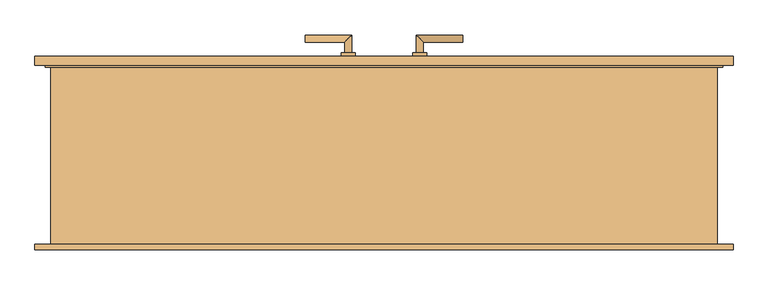
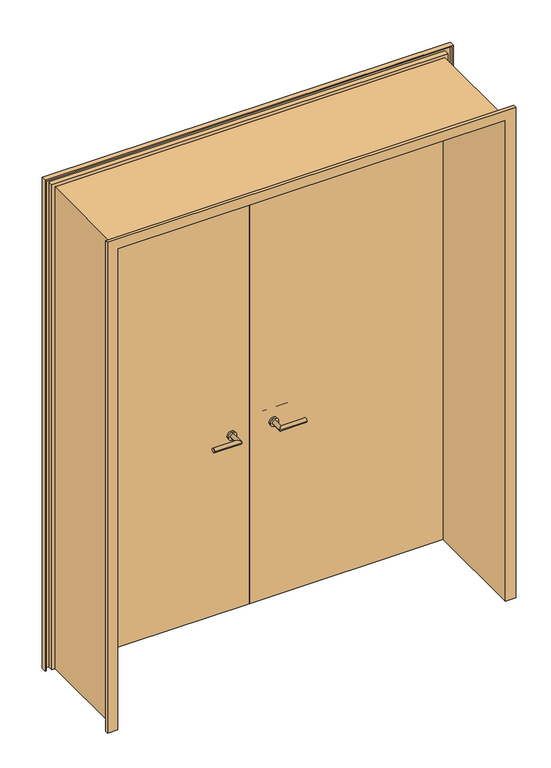
"""IFC4 building model written with IfcOpenShell, lengths in millimetres: door geometry, Drehflügel 2-flg - Stahlzarge : Holztüre 2 flg.1.9x 2.45."""

from ifc_helpers import new_model, si_unit, point, frame, frame_2d, origin, place, context, project, spatial, polyline, circle_curve, ellipse_curve, trimmed, segment, composite_curve, outline, extrude, faceted_brep, source, transform, mapped, element, save
from ifc_brep_helpers import plane_surface, cylinder_surface, advanced_brep


def door_70b3f378(model_context):
    return source(origin(), model_context, "Body", "SolidModel", [
        advanced_brep(
        [(-90.0, 239.4346141, 1000.0), (-110.0, 239.4346141, 1000.0), (-110.0, 189.4346141, 1000.0), (-90.0, 169.4346141, 1000.0), (-220.0, 169.4346141, 1000.0), (-220.0, 189.4346141, 1000.0)],
        [
            (0, 1, circle_curve(frame((-100.0, 239.4346141, 1000.0), z_axis=(0.0, 1.0, 0.0), x_axis=(-1.0, 0.0, 0.0)), 10.0)),
            (1, 0, circle_curve(frame((-100.0, 239.4346141, 1000.0), z_axis=(0.0, 1.0, 0.0), x_axis=(-1.0, 0.0, 0.0)), 10.0)),
            (1, 2),
            (2, 3, ellipse_curve(frame((-100.0, 179.4346141, 1000.0), z_axis=(0.7071067811865385, 0.7071067811865565, 0.0), x_axis=(-0.7071067811865563, 0.7071067811865386, 0.0)), 14.1421356, 10.0)),
            (3, 0),
            (3, 2, ellipse_curve(frame((-100.0, 179.4346141, 1000.0), z_axis=(0.7071067811865385, 0.7071067811865565, 0.0), x_axis=(-0.7071067811865563, 0.7071067811865386, 0.0)), 14.1421356, 10.0)),
            (4, 5, circle_curve(frame((-220.0, 179.4346141, 1000.0), z_axis=(-1.0, 0.0, 0.0), x_axis=(0.0, 1.0, 0.0)), 10.0)),
            (5, 4, circle_curve(frame((-220.0, 179.4346141, 1000.0), z_axis=(-1.0, 0.0, 0.0), x_axis=(0.0, 1.0, 0.0)), 10.0)),
            (2, 5),
            (4, 3),
        ],
        [
            plane_surface(frame((-100.0, 239.4346141, -287.7526403), z_axis=(0.0, 1.0, 0.0), x_axis=(0.0, 0.0, 1.0))),
            cylinder_surface(frame((-100.0, 239.4346141, 1000.0), z_axis=(0.0, 1.0, 0.0), x_axis=(-1.0, 0.0, 0.0)), 10.0),
            plane_surface(frame((-220.0, 179.4346141, -287.7526403), z_axis=(-1.0, 0.0, 0.0), x_axis=(0.0, 0.0, 1.0))),
            cylinder_surface(frame((-100.0, 179.4346141, 1000.0), z_axis=(1.0, 0.0, 0.0), x_axis=(0.0, 1.0, 0.0)), 10.0),
        ],
        [
            (0, [[1, 2]]),
            (1, [[3, 4, 5, -2]]),
            (1, [[-5, 6, -3, -1]]),
            (2, [[7, 8]]),
            (3, [[9, -7, 10, -4]]),
            (3, [[-10, -8, -9, -6]]),
        ],
    ),
        advanced_brep(
        [(-110.0, 299.4346141, 1000.0), (-90.0, 299.4346141, 1000.0), (-90.0, 349.4346141, 1000.0), (-110.0, 329.4346141, 1000.0), (-220.0, 329.4346141, 1000.0), (-220.0, 349.4346141, 1000.0)],
        [
            (0, 1, circle_curve(frame((-100.0, 299.4346141, 1000.0), z_axis=(0.0, -1.0, 0.0), x_axis=(1.0, 0.0, 0.0)), 10.0)),
            (1, 0, circle_curve(frame((-100.0, 299.4346141, 1000.0), z_axis=(0.0, -1.0, 0.0), x_axis=(1.0, 0.0, 0.0)), 10.0)),
            (1, 2),
            (2, 3, ellipse_curve(frame((-100.0, 339.4346141, 1000.0), z_axis=(0.7071067811865475, -0.7071067811865475, 0.0), x_axis=(-0.7071067811865474, -0.7071067811865476, 0.0)), 14.1421356, 10.0)),
            (3, 0),
            (3, 2, ellipse_curve(frame((-100.0, 339.4346141, 1000.0), z_axis=(0.7071067811865475, -0.7071067811865475, 0.0), x_axis=(-0.7071067811865474, -0.7071067811865476, 0.0)), 14.1421356, 10.0)),
            (4, 5, circle_curve(frame((-220.0, 339.4346141, 1000.0), z_axis=(-1.0, 0.0, 0.0), x_axis=(0.0, 1.0, 0.0)), 10.0)),
            (5, 4, circle_curve(frame((-220.0, 339.4346141, 1000.0), z_axis=(-1.0, 0.0, 0.0), x_axis=(0.0, 1.0, 0.0)), 10.0)),
            (2, 5),
            (4, 3),
        ],
        [
            plane_surface(frame((-100.0, 299.4346141, -287.7526403), z_axis=(0.0, -1.0, 0.0), x_axis=(0.0, 0.0, 1.0))),
            cylinder_surface(frame((-100.0, 299.4346141, 1000.0), z_axis=(0.0, -1.0, 0.0), x_axis=(1.0, 0.0, 0.0)), 10.0),
            plane_surface(frame((-220.0, 339.4346141, -287.7526403), z_axis=(-1.0, 0.0, 0.0), x_axis=(0.0, 0.0, 1.0))),
            cylinder_surface(frame((-100.0, 339.4346141, 1000.0), z_axis=(1.0, 0.0, 0.0), x_axis=(0.0, 1.0, 0.0)), 10.0),
        ],
        [
            (0, [[1, 2]]),
            (1, [[3, 4, 5, -2]]),
            (1, [[-5, 6, -3, -1]]),
            (2, [[7, 8]]),
            (3, [[9, -7, 10, -4]]),
            (3, [[-10, -8, -9, -6]]),
        ],
    ),
        extrude(outline(composite_curve([segment(trimmed(circle_curve(frame_2d((1000.0, -100.0)), 20.0), [point((1000.0, -80.0))], [point((1000.0, -120.0))], False, "CARTESIAN"), True, "CONTINUOUS"), segment(trimmed(circle_curve(frame_2d((1000.0, -100.0)), 20.0), [point((1000.0, -120.0))], [point((1000.0, -80.0))], False, "CARTESIAN"), True, "CONTINUOUS")], self_intersect=False)), frame((0.0, 229.4346141, 0.0), z_axis=(0.0, 1.0, 0.0), x_axis=(0.0, 0.0, 1.0)), (0.0, 0.0, 1.0), 10.0),
        extrude(outline(composite_curve([segment(trimmed(circle_curve(frame_2d((1000.0, -100.0)), 20.0), [point((1000.0, -80.0))], [point((1000.0, -120.0))], False, "CARTESIAN"), True, "CONTINUOUS"), segment(trimmed(circle_curve(frame_2d((1000.0, -100.0)), 20.0), [point((1000.0, -120.0))], [point((1000.0, -80.0))], False, "CARTESIAN"), True, "CONTINUOUS")], self_intersect=False)), frame((0.0, 289.4346141, 0.0), z_axis=(0.0, 1.0, 0.0), x_axis=(0.0, 0.0, 1.0)), (0.0, 0.0, 1.0), 10.0),
        advanced_brep(
        [(90.0, 239.4346141, 1000.0), (110.0, 239.4346141, 1000.0), (90.0, 169.4346141, 1000.0), (110.0, 189.4346141, 1000.0), (220.0, 169.4346141, 1000.0), (220.0, 189.4346141, 1000.0)],
        [
            (0, 1, circle_curve(frame((100.0, 239.4346141, 1000.0), z_axis=(0.0, 1.0, 0.0), x_axis=(1.0, 0.0, 0.0)), 10.0)),
            (1, 0, circle_curve(frame((100.0, 239.4346141, 1000.0), z_axis=(0.0, 1.0, 0.0), x_axis=(1.0, 0.0, 0.0)), 10.0)),
            (0, 2),
            (2, 3, ellipse_curve(frame((100.0, 179.4346141, 1000.0), z_axis=(-0.7071067811865385, 0.7071067811865565, 0.0), x_axis=(0.7071067811865563, 0.7071067811865386, 0.0)), 14.1421356, 10.0)),
            (3, 1),
            (3, 2, ellipse_curve(frame((100.0, 179.4346141, 1000.0), z_axis=(-0.7071067811865385, 0.7071067811865565, 0.0), x_axis=(0.7071067811865563, 0.7071067811865386, 0.0)), 14.1421356, 10.0)),
            (4, 5, circle_curve(frame((220.0, 179.4346141, 1000.0), z_axis=(1.0, 0.0, 0.0), x_axis=(0.0, 1.0, 0.0)), 10.0)),
            (5, 4, circle_curve(frame((220.0, 179.4346141, 1000.0), z_axis=(1.0, 0.0, 0.0), x_axis=(0.0, 1.0, 0.0)), 10.0)),
            (2, 4),
            (5, 3),
        ],
        [
            plane_surface(frame((100.0, 239.4346141, -287.7526403), z_axis=(0.0, 1.0, 0.0), x_axis=(0.0, 0.0, 1.0))),
            cylinder_surface(frame((100.0, 239.4346141, 1000.0), z_axis=(0.0, 1.0, 0.0), x_axis=(1.0, 0.0, 0.0)), 10.0),
            plane_surface(frame((220.0, 179.4346141, -287.7526403), z_axis=(1.0, 0.0, 0.0), x_axis=(0.0, 0.0, 1.0))),
            cylinder_surface(frame((100.0, 179.4346141, 1000.0), z_axis=(-1.0, 0.0, 0.0), x_axis=(0.0, 1.0, 0.0)), 10.0),
        ],
        [
            (0, [[1, 2]]),
            (1, [[-1, 3, 4, 5]]),
            (1, [[-2, -5, 6, -3]]),
            (2, [[7, 8]]),
            (3, [[-4, 9, -8, 10]]),
            (3, [[-6, -10, -7, -9]]),
        ],
    ),
        advanced_brep(
        [(110.0, 299.4346141, 1000.0), (90.0, 299.4346141, 1000.0), (110.0, 329.4346141, 1000.0), (90.0, 349.4346141, 1000.0), (220.0, 329.4346141, 1000.0), (220.0, 349.4346141, 1000.0)],
        [
            (0, 1, circle_curve(frame((100.0, 299.4346141, 1000.0), z_axis=(0.0, -1.0, 0.0), x_axis=(-1.0, 0.0, 0.0)), 10.0)),
            (1, 0, circle_curve(frame((100.0, 299.4346141, 1000.0), z_axis=(0.0, -1.0, 0.0), x_axis=(-1.0, 0.0, 0.0)), 10.0)),
            (0, 2),
            (2, 3, ellipse_curve(frame((100.0, 339.4346141, 1000.0), z_axis=(-0.7071067811865475, -0.7071067811865475, 0.0), x_axis=(0.7071067811865474, -0.7071067811865476, 0.0)), 14.1421356, 10.0)),
            (3, 1),
            (3, 2, ellipse_curve(frame((100.0, 339.4346141, 1000.0), z_axis=(-0.7071067811865475, -0.7071067811865475, 0.0), x_axis=(0.7071067811865474, -0.7071067811865476, 0.0)), 14.1421356, 10.0)),
            (4, 5, circle_curve(frame((220.0, 339.4346141, 1000.0), z_axis=(1.0, 0.0, 0.0), x_axis=(0.0, 1.0, 0.0)), 10.0)),
            (5, 4, circle_curve(frame((220.0, 339.4346141, 1000.0), z_axis=(1.0, 0.0, 0.0), x_axis=(0.0, 1.0, 0.0)), 10.0)),
            (2, 4),
            (5, 3),
        ],
        [
            plane_surface(frame((100.0, 299.4346141, -287.7526403), z_axis=(0.0, -1.0, 0.0), x_axis=(0.0, 0.0, 1.0))),
            cylinder_surface(frame((100.0, 299.4346141, 1000.0), z_axis=(0.0, -1.0, 0.0), x_axis=(-1.0, 0.0, 0.0)), 10.0),
            plane_surface(frame((220.0, 339.4346141, -287.7526403), z_axis=(1.0, 0.0, 0.0), x_axis=(0.0, 0.0, 1.0))),
            cylinder_surface(frame((100.0, 339.4346141, 1000.0), z_axis=(-1.0, 0.0, 0.0), x_axis=(0.0, 1.0, 0.0)), 10.0),
        ],
        [
            (0, [[1, 2]]),
            (1, [[-1, 3, 4, 5]]),
            (1, [[-2, -5, 6, -3]]),
            (2, [[7, 8]]),
            (3, [[-4, 9, -8, 10]]),
            (3, [[-6, -10, -7, -9]]),
        ],
    ),
        extrude(outline(composite_curve([segment(trimmed(circle_curve(frame_2d((1000.0, 100.0)), 20.0), [point((1000.0, 80.0))], [point((1000.0, 120.0))], False, "CARTESIAN"), True, "CONTINUOUS"), segment(trimmed(circle_curve(frame_2d((1000.0, 100.0)), 20.0), [point((1000.0, 120.0))], [point((1000.0, 80.0))], False, "CARTESIAN"), True, "CONTINUOUS")], self_intersect=False)), frame((0.0, 229.4346141, 0.0), z_axis=(0.0, 1.0, 0.0), x_axis=(0.0, 0.0, 1.0)), (0.0, 0.0, 1.0), 10.0),
        extrude(outline(composite_curve([segment(trimmed(circle_curve(frame_2d((1000.0, 100.0)), 20.0), [point((1000.0, 80.0))], [point((1000.0, 120.0))], False, "CARTESIAN"), True, "CONTINUOUS"), segment(trimmed(circle_curve(frame_2d((1000.0, 100.0)), 20.0), [point((1000.0, 120.0))], [point((1000.0, 80.0))], False, "CARTESIAN"), True, "CONTINUOUS")], self_intersect=False)), frame((0.0, 289.4346141, 0.0), z_axis=(0.0, 1.0, 0.0), x_axis=(0.0, 0.0, 1.0)), (0.0, 0.0, 1.0), 10.0),
        extrude(outline(polyline([(0.0, 264.4346141), (-940.0, 264.4346141), (-940.0, 289.4346141), (0.0, 289.4346141), (0.0, 264.4346141)])), frame((0.0, 0.0, 100.0), z_axis=(0.0, 0.0, 1.0), x_axis=(1.0, 0.0, 0.0)), (0.0, 0.0, 1.0), 2440.0),
        extrude(outline(polyline([(940.0, 264.4346141), (0.0, 264.4346141), (0.0, 289.4346141), (940.0, 289.4346141), (940.0, 264.4346141)])), frame((0.0, 0.0, 100.0), z_axis=(0.0, 0.0, 1.0), x_axis=(1.0, 0.0, 0.0)), (0.0, 0.0, 1.0), 2440.0),
        faceted_brep([(974.5, -250.5653859, 100.0), (925.0, -250.5653859, 100.0), (925.0, 264.4346141, 100.0), (940.0, 264.4346141, 100.0), (940.0, 289.4346141, 100.0), (974.5, 289.4346141, 100.0), (974.5, 264.4346141, 100.0), (969.5, 264.4346141, 100.0), (969.5, 284.4346141, 100.0), (945.0, 284.4346141, 100.0), (945.0, 259.4346141, 100.0), (930.0, 259.4346141, 100.0), (930.0, -245.5653859, 100.0), (969.5, -245.5653859, 100.0), (969.5, -235.5653859, 100.0), (974.5, -235.5653859, 100.0), (974.5, -250.5653859, 2574.5), (-974.5, -250.5653859, 2574.5), (-974.5, -250.5653859, 100.0), (-925.0, -250.5653859, 100.0), (-925.0, -250.5653859, 2525.0), (925.0, -250.5653859, 2525.0), (925.0, 264.4346141, 2525.0), (-925.0, 264.4346141, 2525.0), (-925.0, 264.4346141, 100.0), (-940.0, 264.4346141, 100.0), (-940.0, 264.4346141, 2540.0), (940.0, 264.4346141, 2540.0), (940.0, 289.4346141, 2540.0), (-940.0, 289.4346141, 2540.0), (-940.0, 289.4346141, 100.0), (-974.5, 289.4346141, 100.0), (-974.5, 289.4346141, 2574.5), (974.5, 289.4346141, 2574.5), (974.5, 264.4346141, 2574.5), (-974.5, 264.4346141, 2574.5), (-974.5, 264.4346141, 100.0), (-969.5, 264.4346141, 100.0), (-969.5, 264.4346141, 2569.5), (969.5, 264.4346141, 2569.5), (969.5, 284.4346141, 2569.5), (-969.5, 284.4346141, 2569.5), (-969.5, 284.4346141, 100.0), (-945.0, 284.4346141, 100.0), (-945.0, 284.4346141, 2545.0), (945.0, 284.4346141, 2545.0), (945.0, 259.4346141, 2545.0), (-945.0, 259.4346141, 2545.0), (-945.0, 259.4346141, 100.0), (-930.0, 259.4346141, 100.0), (-930.0, 259.4346141, 2530.0), (930.0, 259.4346141, 2530.0), (930.0, -245.5653859, 2530.0), (-930.0, -245.5653859, 2530.0), (-930.0, -245.5653859, 100.0), (-969.5, -245.5653859, 100.0), (-969.5, -245.5653859, 2569.5), (969.5, -245.5653859, 2569.5), (969.5, -235.5653859, 2569.5), (-969.5, -235.5653859, 2569.5), (-969.5, -235.5653859, 100.0), (-974.5, -235.5653859, 100.0), (-974.5, -235.5653859, 2574.5), (974.5, -235.5653859, 2574.5)], [[[0, 1, 2, 3, 4, 5, 6, 7, 8, 9, 10, 11, 12, 13, 14, 15]], [[1, 0, 16, 17, 18, 19, 20, 21]], [[2, 1, 21, 22]], [[3, 2, 22, 23, 24, 25, 26, 27]], [[4, 3, 27, 28]], [[5, 4, 28, 29, 30, 31, 32, 33]], [[6, 5, 33, 34]], [[7, 6, 34, 35, 36, 37, 38, 39]], [[8, 7, 39, 40]], [[9, 8, 40, 41, 42, 43, 44, 45]], [[10, 9, 45, 46]], [[11, 10, 46, 47, 48, 49, 50, 51]], [[12, 11, 51, 52]], [[13, 12, 52, 53, 54, 55, 56, 57]], [[14, 13, 57, 58]], [[15, 14, 58, 59, 60, 61, 62, 63]], [[0, 15, 63, 16]], [[17, 62, 61, 18]], [[18, 61, 60, 55, 54, 49, 48, 43, 42, 37, 36, 31, 30, 25, 24, 19]], [[23, 20, 19, 24]], [[29, 26, 25, 30]], [[35, 32, 31, 36]], [[41, 38, 37, 42]], [[47, 44, 43, 48]], [[53, 50, 49, 54]], [[59, 56, 55, 60]], [[22, 21, 20, 23]], [[28, 27, 26, 29]], [[34, 33, 32, 35]], [[40, 39, 38, 41]], [[46, 45, 44, 47]], [[52, 51, 50, 53]], [[58, 57, 56, 59]], [[16, 63, 62, 17]]]),
    ])


if __name__ == "__main__":
    model = new_model("IFC4")
    model_context = context("Model", 3, world=origin())
    ifc_project = project(units=[si_unit("LENGTHUNIT", "METRE", prefix="MILLI")], contexts=[model_context])
    site = spatial("IfcSite", under=ifc_project)
    building = spatial("IfcBuilding", under=site)
    placement = place(None, origin())
    door_shape = door_70b3f378(model_context)
    element("IfcDoor", 1, ObjectType="Drehflügel 2-flg - Stahlzarge : Holztüre 2 flg.1.9x 2.45", at=placement, inside=building, context=model_context, shape_type="MappedRepresentation", body=[
        mapped(door_shape, transform((0.0, 0.0, 0.0), x_axis=(1.0, 0.0, 0.0), y_axis=(0.0, 1.0, 0.0), z_axis=(0.0, 0.0, 1.0))),
    ])
    save(model, "model.ifc")

# Revit data of these elements
# Type "Drehflügel 2-flg - Stahlzarge : Holztüre 2 flg.1.9x 2.45"
#   Type Mark = "22"
#   Operation = "DoubleDoorSingleSwing"
#   Keynote = "16.03"
#   Analytic Construction = "Metall"
#   Thermal Resistance (R) = 0.270117 (m²·K)/W
#   Heat Transfer Coefficient (U) = 3.7021 W/(m²·K)
#   Rough Width = 1.900 m
#   Rough Height [instance default] = 2.550 m
#   Höhe Türgriff = 0.900 m
#   Height = 2.450 m
#   Fußbodenaufbau [instance default] = 0.100 m
#   Width = 1.900 m
#   Sichtbarkeit Sturzlinien [instance default] = yes
#   Türgriff auswählen [instance default] = element 219327
#   Türgriff [instance default] = none
#   Türflügel [instance default] = none
#   Rahmen/Pfosten [instance default] = Metall - Lackiert - Grau
#   Visual Light Transmittance = 0
#   Solar Heat Gain Coefficient = 0
#   Function = (empty or 0)
#   Wall Closure = (empty or 0)
# Element 1 (IfcDoor, "Drehflügel 2-flg - Stahlzarge : Holztüre 2 flg.1.9x 2.45")
#   Rahmen/Pfosten = Holz - Eiche
#   Materials on its faces: "Metall - Chrom", "Holz - Eiche", "Holz - Birke"
# Materials
#   "Metall - Lackiert - Grau": class "Farbe 1", colour RGB 98 98 98, transparency 0, Cost = 0
#   "Metall - Chrom": class "Metall", colour RGB 247 247 247, transparency 0, Cost = 0
#   "Holz - Eiche": class "Holz", colour RGB 151 89 53, transparency 0, Cost = 0
#   "Holz - Birke": class "Holz", colour RGB 213 164 103, transparency 0, Cost = 0
